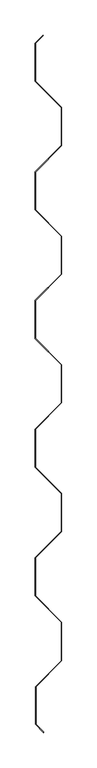
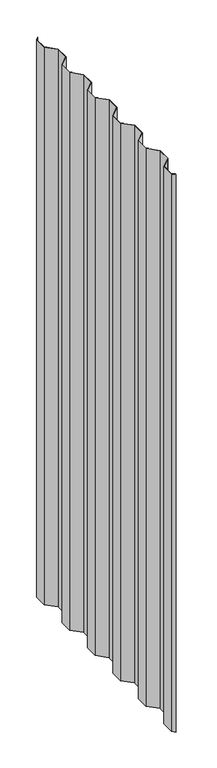
"""IFC4 building model written with IfcOpenShell, lengths in millimetres: proxy geometry, MBCI 7.2-V Panel18 : MBCI 7.2-V Panel-1."""

from ifc_helpers import new_model, si_unit, origin, origin_with_axes, place, context, project, spatial, polyline, outline, extrude, source, transform, mapped, element, save


def generic_models_435dda05(model_context):
    return source(origin(), model_context, "Body", "SweptSolid", [
        extrude(outline(polyline([(590353.5827614, -535268.7919067), (590353.5827614, -535214.6801976), (590364.9833956, -535203.2795634), (590365.0253204, -535204.0795376), (590354.1780739, -535214.9267841), (590354.1780739, -535268.5453202), (590391.6684739, -535306.0357202), (590391.6684739, -535360.3163841), (590354.1780739, -535397.8067841), (590354.1780739, -535451.4253202), (590391.6684739, -535488.9157202), (590391.6684739, -535543.1963841), (590354.1780739, -535580.6867841), (590354.1780739, -535634.3053202), (590391.6684739, -535671.7957202), (590391.6684739, -535726.0763841), (590354.1780739, -535763.5667841), (590354.1780739, -535817.1853202), (590391.6684739, -535854.6757202), (590391.6684739, -535908.9563841), (590354.1780739, -535946.4467841), (590354.1780739, -536000.0653202), (590391.6684739, -536037.5557202), (590391.6684739, -536092.6999841), (590354.7876739, -536129.5807841), (590354.7876739, -536182.6689111), (590365.9181078, -536193.799345), (590365.8630841, -536194.5862203), (590354.1923614, -536182.9154976), (590354.1923614, -536129.3341976), (590391.0731614, -536092.4533976), (590391.0731614, -536037.8023067), (590353.5827614, -536000.3119067), (590353.5827614, -535946.2001976), (590391.0731614, -535908.7097976), (590391.0731614, -535854.9223067), (590353.5827614, -535817.4319067), (590353.5827614, -535763.3201976), (590391.0731614, -535725.8297976), (590391.0731614, -535672.0423067), (590353.5827614, -535634.5519067), (590353.5827614, -535580.4401976), (590391.0731614, -535542.9497976), (590391.0731614, -535489.1623067), (590353.5827614, -535451.6719067), (590353.5827614, -535397.5601976), (590391.0731614, -535360.0697976), (590391.0731614, -535306.2823067), (590353.5827614, -535268.7919067)])), origin_with_axes(), (0.0, 0.0, 1.0), 2438.4),
    ])


if __name__ == "__main__":
    model = new_model("IFC4")
    model_context = context("Model", 3, world=origin())
    ifc_project = project(units=[si_unit("LENGTHUNIT", "METRE", prefix="MILLI")], contexts=[model_context])
    site = spatial("IfcSite", under=ifc_project)
    building = spatial("IfcBuilding", under=site)
    placement = place(None, origin())
    generic_models_shape = generic_models_435dda05(model_context)
    element("IfcBuildingElementProxy", 1, Name="MBCI 7.2-V Panel18 : MBCI 7.2-V Panel-1", ObjectType="MBCI 7.2-V Panel18 : MBCI 7.2-V Panel-1", at=placement, inside=building, context=model_context, shape_type="MappedRepresentation", body=[
        mapped(generic_models_shape, transform((0.0, 0.0, 0.0), x_axis=(1.0, 0.0, 0.0), y_axis=(0.0, 1.0, 0.0), z_axis=(0.0, 0.0, 1.0))),
    ])
    save(model, "model.ifc")

# Revit data of these elements
# Element 1 (IfcBuildingElementProxy, "MBCI 7.2-V Panel18 : MBCI 7.2-V Panel-1")
#   Materials on its faces: "MTL PANEL"
# Materials
#   "MTL PANEL": class "Generic", colour RGB 239 242 240, transparency 0, Cost = 0
